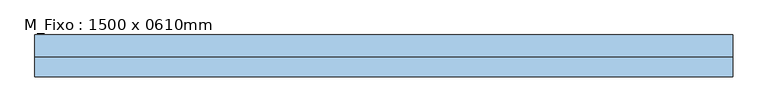
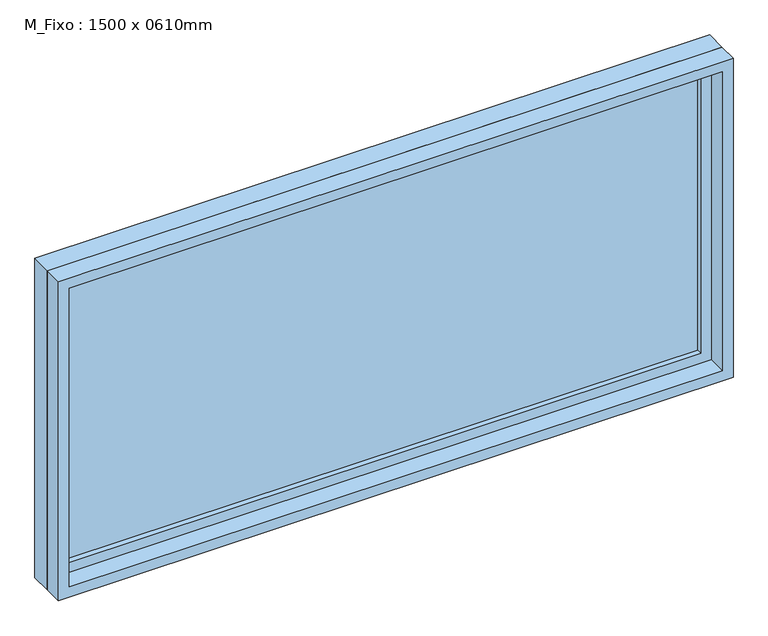
"""IFC4 building model written with IfcOpenShell, lengths in millimetres: window geometry, M_Fixo : 1500 x 0610mm."""

from ifc_helpers import new_model, si_unit, frame, origin, place, context, project, spatial, polyline, outline, extrude, source, transform, mapped, element, save


def m_fixo_1500_x_0610mm_b1555d91(model_context):
    return source(origin(), model_context, "Body", "SweptSolid", [
        extrude(outline(polyline([(-937.0, 38.0), (937.0, 38.0), (937.0, 26.0), (-937.0, 26.0), (-937.0, 38.0)])), frame((0.0, 0.0, 1063.0), z_axis=(0.0, 0.0, 1.0), x_axis=(1.0, 0.0, 0.0)), (0.0, 0.0, 1.0), 874.0),
        extrude(outline(polyline([(1981.0, -981.0), (1019.0, -981.0), (1019.0, 981.0), (1981.0, 981.0), (1981.0, -981.0)]), holes=[polyline([(1937.0, -937.0), (1937.0, 937.0), (1063.0, 937.0), (1063.0, -937.0), (1937.0, -937.0)])]), frame((0.0, 10.0, 0.0), z_axis=(0.0, 1.0, 0.0), x_axis=(0.0, 0.0, 1.0)), (0.0, 0.0, 1.0), 44.0),
        extrude(outline(polyline([(2000.0, -1000.0), (1000.0, -1000.0), (1000.0, 1000.0), (2000.0, 1000.0), (2000.0, -1000.0)]), holes=[polyline([(1981.0, -981.0), (1981.0, 981.0), (1019.0, 981.0), (1019.0, -981.0), (1981.0, -981.0)])]), frame((0.0, 10.0, 0.0), z_axis=(0.0, 1.0, 0.0), x_axis=(0.0, 0.0, 1.0)), (0.0, 0.0, 1.0), 63.0),
        extrude(outline(polyline([(2000.0, -1000.0), (1000.0, -1000.0), (1000.0, 1000.0), (2000.0, 1000.0), (2000.0, -1000.0)]), holes=[polyline([(1968.0, -968.0), (1968.0, 968.0), (1032.0, 968.0), (1032.0, -968.0), (1968.0, -968.0)])]), frame((0.0, -47.0, 0.0), z_axis=(0.0, 1.0, 0.0), x_axis=(0.0, 0.0, 1.0)), (0.0, 0.0, 1.0), 57.0),
    ])


if __name__ == "__main__":
    model = new_model("IFC4")
    model_context = context("Model", 3, world=origin())
    ifc_project = project(units=[si_unit("LENGTHUNIT", "METRE", prefix="MILLI")], contexts=[model_context])
    site = spatial("IfcSite", under=ifc_project)
    building = spatial("IfcBuilding", under=site)
    placement = place(None, origin())
    m_fixo_1500_x_0610mm_shape = m_fixo_1500_x_0610mm_b1555d91(model_context)
    element("IfcWindow", 1, ObjectType="M_Fixo : 1500 x 0610mm", at=placement, inside=building, context=model_context, shape_type="MappedRepresentation", body=[
        mapped(m_fixo_1500_x_0610mm_shape, transform((0.0, 0.0, 0.0), x_axis=(1.0, 0.0, 0.0), y_axis=(0.0, 1.0, 0.0), z_axis=(0.0, 0.0, 1.0))),
    ])
    save(model, "model.ifc")

# Revit data of these elements
# Type "M_Fixo : 1500 x 0610mm"
#   Type Mark = "19"
#   Construction Type Id = "GSP4R"
#   Analytic Construction = "Vidraça única Pilkington 1/8 pol"
#   Visual Light Transmittance = 0.9
#   Thermal Resistance (R) = 0.271106 (m²·K)/W
#   Solar Heat Gain Coefficient = 0.78
#   Heat Transfer Coefficient (U) = 3.6886 W/(m²·K)
#   Height = 1.00 m
#   Altura-padrão do peitoril = 1.00 m
#   Width = 2.00 m
#   Janela aplicada = 0.019 m
#   Define Thermal Properties by = 1
#   Material da estrutura externa = Caixilho
#   Material da estrutura interna = Caixilho
#   Material do painel de vidro = Vidro
#   Caixilho = Caixilho
#   Wall Closure = (empty or 0)
# Element 1 (IfcWindow, "M_Fixo : 1500 x 0610mm")
#   Materials on its faces: "Caixilho", "Vidro"
# Materials
#   "Caixilho": class "Madeira", colour RGB 224 178 126, transparency 0, Cost = 0
#   "Vidro": class "Vidro", colour RGB 0 128 192, transparency 0.9, Description = "Vidro de sílica", Cost = 0
